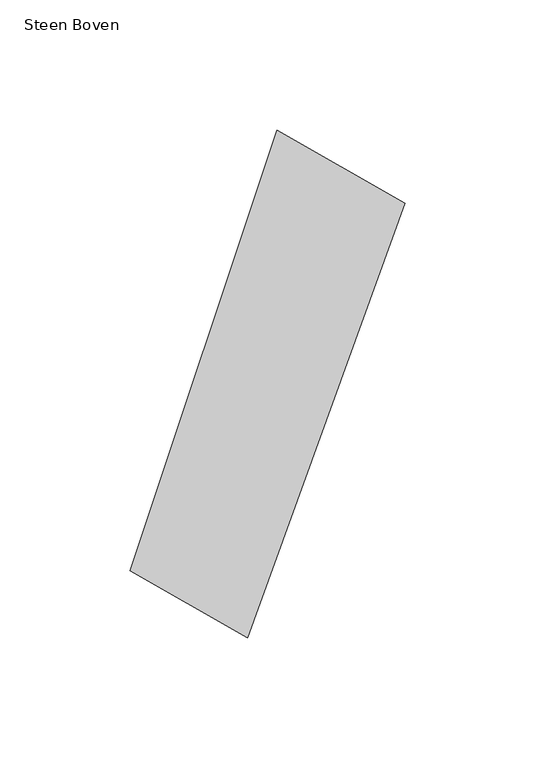
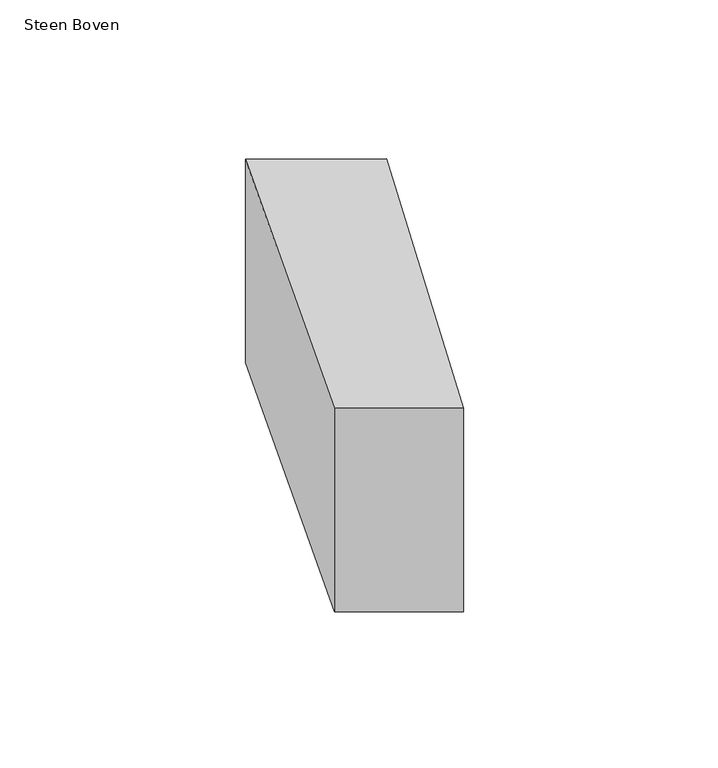
"""IFC4 building model written with IfcOpenShell, lengths in millimetres: proxy geometry, 00_GMA_steen_versie_4 : Steen Boven."""

from ifc_helpers import new_model, si_unit, origin, origin_with_axes, place, context, project, spatial, polyline, outline, extrude, source, transform, mapped, element, save


def steen_boven_1dfbeaee(model_context):
    return source(origin(), model_context, "Body", "SweptSolid", [
        extrude(outline(polyline([(132.3657516, 156.9447185), (71.764981, -10.0876563), (26.6257123, 15.7145055), (83.1799269, 185.0848281), (132.3657516, 156.9447185)])), origin_with_axes(), (0.0, 0.0, 1.0), 100.0),
    ])


if __name__ == "__main__":
    model = new_model("IFC4")
    model_context = context("Model", 3, world=origin())
    ifc_project = project(units=[si_unit("LENGTHUNIT", "METRE", prefix="MILLI")], contexts=[model_context])
    site = spatial("IfcSite", under=ifc_project)
    building = spatial("IfcBuilding", under=site)
    placement = place(None, origin())
    steen_boven_shape = steen_boven_1dfbeaee(model_context)
    element("IfcBuildingElementProxy", 1, Name="00_GMA_steen_versie_4 : Steen Boven", ObjectType="00_GMA_steen_versie_4 : Steen Boven", at=placement, inside=building, context=model_context, shape_type="MappedRepresentation", body=[
        mapped(steen_boven_shape, transform((0.0, 0.0, 0.0), x_axis=(1.0, 0.0, 0.0), y_axis=(0.0, 1.0, 0.0), z_axis=(0.0, 0.0, 1.0))),
    ])
    save(model, "model.ifc")

# Revit data of these elements
# Type "00_GMA_steen_versie_4 : Steen Boven"
#   StootVoegHalfBoven [instance default] = 5 mm
#   StootVoegHalf [instance default] = 5 mm
#   StootVoegBreedteOnder = 10 mm
#   StootVoegBreedteBoven = 10 mm
#   Steendikte = 100 mm
#   LintVoegOnderHalf = 5 mm
#   LintVoegOnder = 10 mm
#   LintVoegBovenHalf = 0 mm
#   LintVoegBoven = 0 mm
#   materiaal = none
#   MateriaalVoeg = none
#   Default Elevation = 0
